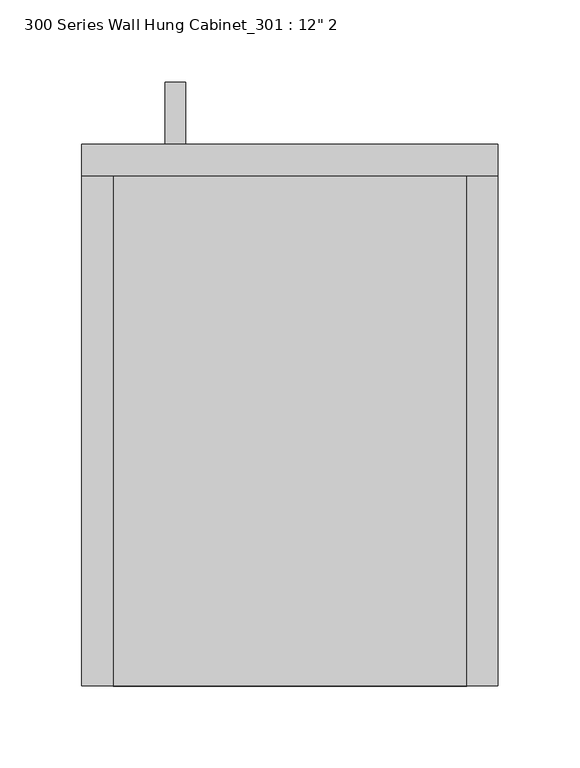
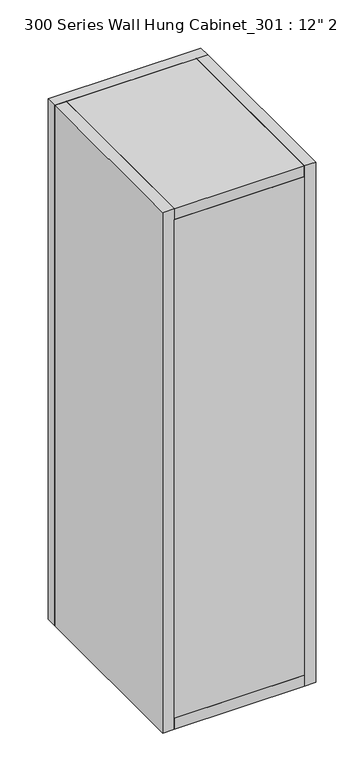
"""IFC4 building model written with IfcOpenShell, lengths in millimetres: furniture geometry."""

import ifcopenshell
import ifcopenshell.guid

model = None  # the IFC model being written
_history = None  # IfcOwnerHistory: only IFC2X3 demands one
_inside = {}  # id of a spatial element -> (the spatial element, [elements in it])
_under = {}  # id of a project, library or spatial element -> (it, [spatial elements below it])
_declared = {}  # id of a project -> (the project, [libraries it declares])
_typed = {}  # id of a type object -> (the type object, [elements of that type])
_made_of = {}  # id of a material, layer set ... -> (it, [elements and type objects made of it])


def new_model(schema):
    """Start an empty IFC model of exactly this schema.

    Asked for "IFC4X3", IfcOpenShell would pick the latest addendum, in which some entities
    have other attributes; the version numbers below select the first issue.
    IFC2X3 requires an IfcOwnerHistory on every rooted entity: one is made here for all.
    """
    global model, _history
    if schema == "IFC4X3":
        model = ifcopenshell.file(schema_version=(4, 3, 0, 0))
    else:
        model = ifcopenshell.file(schema=schema)
    _inside.clear()
    _under.clear()
    _declared.clear()
    _typed.clear()
    _made_of.clear()
    _history = None
    if model.schema == "IFC2X3":
        org = make("IfcOrganization", Name="unknown")
        user = make(
            "IfcPersonAndOrganization",
            ThePerson=make("IfcPerson", FamilyName="unknown"),
            TheOrganization=org,
        )
        app = make(
            "IfcApplication",
            ApplicationDeveloper=org,
            Version="unknown",
            ApplicationFullName="unknown",
            ApplicationIdentifier="unknown",
        )
        _history = make(
            "IfcOwnerHistory",
            OwningUser=user,
            OwningApplication=app,
            ChangeAction="ADDED",
            CreationDate=0,
        )
    return model


def make(cls, **values):
    """One entity of the class cls with the attributes given. An attribute that is None is left unset."""
    return model.create_entity(
        cls, **{name: value for name, value in values.items() if value is not None}
    )


def rooted(cls, **values):
    """An entity with a GlobalId (a new one), such as an element, a storey or a relation."""
    return make(cls, GlobalId=ifcopenshell.guid.new(), OwnerHistory=_history, **values)


def si_unit(unit_type, name, prefix=None):
    """IfcSIUnit, for example si_unit("LENGTHUNIT", "METRE", prefix="MILLI")."""
    return make("IfcSIUnit", UnitType=unit_type, Prefix=prefix, Name=name)


def assignment(units):
    """IfcUnitAssignment: the units of a project."""
    return None if units is None else make("IfcUnitAssignment", Units=units)


def point(xyz):
    """IfcCartesianPoint."""
    return None if xyz is None else make("IfcCartesianPoint", Coordinates=xyz)


def direction(xyz):
    """IfcDirection."""
    return None if xyz is None else make("IfcDirection", DirectionRatios=xyz)


def frame(location, z_axis=None, x_axis=None):
    """IfcAxis2Placement3D, a coordinate frame: its origin and axes. An axis left out is left unset."""
    return make(
        "IfcAxis2Placement3D",
        Location=point(location),
        Axis=direction(z_axis),
        RefDirection=direction(x_axis),
    )


def origin():
    """The frame at (0, 0, 0) with its axes left unset."""
    return frame((0.0, 0.0, 0.0))


def place(relative_to, where):
    """IfcLocalPlacement: puts the frame where relative to a parent placement (None: the world)."""
    return make(
        "IfcLocalPlacement", PlacementRelTo=relative_to, RelativePlacement=where
    )


def context(
    kind, dimensions, precision=None, world=None, true_north=None, identifier=None
):
    """IfcGeometricRepresentationContext, for example the 3D "Model" context."""
    return make(
        "IfcGeometricRepresentationContext",
        ContextIdentifier=identifier,
        ContextType=kind,
        CoordinateSpaceDimension=dimensions,
        Precision=precision,
        WorldCoordinateSystem=world,
        TrueNorth=true_north,
    )


def project(units=None, contexts=None):
    """IfcProject with its units and contexts."""
    return rooted(
        "IfcProject",
        Name="project",
        RepresentationContexts=contexts,
        UnitsInContext=assignment(units),
    )


def spatial(cls, under=None, at=None, **own):
    """A site, building, storey or space (cls), placed at a placement, below another one or the project."""
    s = rooted(cls, ObjectPlacement=at, **own)
    if under is not None:
        _under.setdefault(under.id(), (under, []))[1].append(s)
    return s


def polyline(points):
    """IfcPolyline through the points."""
    return make("IfcPolyline", Points=[point(p) for p in points])


def outline(outer, holes=None, kind="AREA"):
    """IfcArbitraryClosedProfileDef: a profile drawn as a closed curve; with holes, ...WithVoids."""
    if holes is None:
        return make("IfcArbitraryClosedProfileDef", ProfileType=kind, OuterCurve=outer)
    return make(
        "IfcArbitraryProfileDefWithVoids",
        ProfileType=kind,
        OuterCurve=outer,
        InnerCurves=holes,
    )


def extrude(swept, where, along, depth):
    """IfcExtrudedAreaSolid: the profile swept, set in the frame where, extruded along a direction by depth."""
    return make(
        "IfcExtrudedAreaSolid",
        SweptArea=swept,
        Position=where,
        ExtrudedDirection=direction(along),
        Depth=depth,
    )


def shape(context_of_items, identifier, shape_type, items):
    """IfcShapeRepresentation: the items that make up one representation, for example the "Body"."""
    return make(
        "IfcShapeRepresentation",
        ContextOfItems=context_of_items,
        RepresentationIdentifier=identifier,
        RepresentationType=shape_type,
        Items=items,
    )


def source(mapping_origin, context_of_items, identifier, shape_type, items):
    """IfcRepresentationMap: a shape defined once, which mapped items show again and again."""
    return make(
        "IfcRepresentationMap",
        MappingOrigin=mapping_origin,
        MappedRepresentation=shape(context_of_items, identifier, shape_type, items),
    )


def transform(
    local_origin,
    x_axis=None,
    y_axis=None,
    z_axis=None,
    scale=None,
    scale2=None,
    scale3=None,
    uniform=True,
):
    """IfcCartesianTransformationOperator3D, or its non-uniform kind. x_axis, y_axis, z_axis: its Axis1, 2, 3."""
    if uniform:
        return make(
            "IfcCartesianTransformationOperator3D",
            Axis1=direction(x_axis),
            Axis2=direction(y_axis),
            LocalOrigin=point(local_origin),
            Scale=scale,
            Axis3=direction(z_axis),
        )
    return make(
        "IfcCartesianTransformationOperator3DnonUniform",
        Axis1=direction(x_axis),
        Axis2=direction(y_axis),
        LocalOrigin=point(local_origin),
        Scale=scale,
        Axis3=direction(z_axis),
        Scale2=scale2,
        Scale3=scale3,
    )


def mapped(mapping_source, mapping_target):
    """IfcMappedItem: shows the shape of a source again, moved by a transform."""
    return make(
        "IfcMappedItem", MappingSource=mapping_source, MappingTarget=mapping_target
    )


def made_of(thing, what):
    """Note that an element or type object is made of a material, layer set ...; save() writes the relation."""
    if what is not None:
        _made_of.setdefault(what.id(), (what, []))[1].append(thing)
    return thing


def element(
    cls,
    number,
    at=None,
    inside=None,
    cuts=None,
    type_object=None,
    material=None,
    context=None,
    identifier="Body",
    shape_type=None,
    held_by="IfcProductDefinitionShape",
    body=None,
    shapes=None,
    **own,
):
    """One element of the class cls, such as IfcWall. Its Tag is "e" and its number.

    at: its placement. inside: the storey or other place that contains it. cuts: it is an
    opening in that element (IfcRelVoidsElement). A single representation is given by context,
    identifier, shape_type and body (its items); several are given by shapes. held_by: the class
    of the entity that holds the representations. save() writes the other relations.
    """
    e = rooted(cls, Tag="e%d" % number, ObjectPlacement=at, **own)
    if body is not None:
        shapes = [shape(context, identifier, shape_type, body)]
    if shapes is not None:
        e.Representation = make(held_by, Representations=shapes)
    if inside is not None:
        _inside.setdefault(inside.id(), (inside, []))[1].append(e)
    if cuts is not None:
        rooted(
            "IfcRelVoidsElement", RelatingBuildingElement=cuts, RelatedOpeningElement=e
        )
    if type_object is not None:
        _typed.setdefault(type_object.id(), (type_object, []))[1].append(e)
    return made_of(e, material)


def aggregate(whole, parts):
    """IfcRelAggregates: a whole, such as a stair, and the parts it consists of."""
    return rooted("IfcRelAggregates", RelatingObject=whole, RelatedObjects=parts)


def save(model, path):
    """Write the relations noted so far, then the file.

    IfcRelAggregates (storeys below a building ...), IfcRelContainedInSpatialStructure (elements
    in a storey), IfcRelDefinesByType, IfcRelAssociatesMaterial and IfcRelDeclares: one each for
    every whole, place, type object, material and project.
    """
    for whole, parts in _under.values():
        aggregate(whole, parts)
    for where, things in _inside.values():
        rooted(
            "IfcRelContainedInSpatialStructure",
            RelatedElements=things,
            RelatingStructure=where,
        )
    for kind, things in _typed.values():
        rooted("IfcRelDefinesByType", RelatedObjects=things, RelatingType=kind)
    for what, things in _made_of.values():
        rooted("IfcRelAssociatesMaterial", RelatedObjects=things, RelatingMaterial=what)
    for by, libraries in _declared.values():
        rooted("IfcRelDeclares", RelatingContext=by, RelatedDefinitions=libraries)
    model.write(path)


def furniture_bfdc1b7c(model_context):
    return source(origin(), model_context, "Body", "SweptSolid", [
        extrude(outline(polyline([(406.4, 1352.5425373), (406.4, 1365.2121874), (444.4810937, 1365.2121874), (444.4810937, 1270.0), (406.4, 1270.0), (406.4, 1282.6696501), (431.8114436, 1282.6696501), (431.8114436, 1352.5425373), (406.4, 1352.5425373)])), frame((-76.2, 0.0, 0.0), z_axis=(1.0, 0.0, 0.0), x_axis=(0.0, 1.0, 0.0)), (0.0, 0.0, 1.0), 12.4065288),
        extrude(outline(polyline([(107.95, 387.35), (107.95, 76.2), (-107.95, 76.2), (-107.95, 387.35), (107.95, 387.35)])), frame((0.0, 0.0, 1219.2), z_axis=(0.0, 0.0, 1.0), x_axis=(1.0, 0.0, 0.0)), (0.0, 0.0, 1.0), 19.05),
        extrude(outline(polyline([(107.95, 76.2), (-107.95, 76.2), (-107.95, 95.25), (107.95, 95.25), (107.95, 76.2)])), frame((0.0, 0.0, 1238.25), z_axis=(0.0, 0.0, 1.0), x_axis=(1.0, 0.0, 0.0)), (0.0, 0.0, 1.0), 876.3),
        extrude(outline(polyline([(127.0, 387.35), (-127.0, 387.35), (-127.0, 406.4), (127.0, 406.4), (127.0, 387.35)])), frame((0.0, 0.0, 1219.2), z_axis=(0.0, 0.0, 1.0), x_axis=(1.0, 0.0, 0.0)), (0.0, 0.0, 1.0), 914.4),
        extrude(outline(polyline([(-127.0, 76.2), (-127.0, 387.35), (-107.95, 387.35), (-107.95, 76.2), (-127.0, 76.2)])), frame((0.0, 0.0, 1219.2), z_axis=(0.0, 0.0, 1.0), x_axis=(1.0, 0.0, 0.0)), (0.0, 0.0, 1.0), 914.4),
        extrude(outline(polyline([(107.95, 76.2), (107.95, 387.35), (127.0, 387.35), (127.0, 76.2), (107.95, 76.2)])), frame((0.0, 0.0, 1219.2), z_axis=(0.0, 0.0, 1.0), x_axis=(1.0, 0.0, 0.0)), (0.0, 0.0, 1.0), 914.4),
        extrude(outline(polyline([(107.95, 387.35), (107.95, 76.2), (-107.95, 76.2), (-107.95, 387.35), (107.95, 387.35)])), frame((0.0, 0.0, 2114.55), z_axis=(0.0, 0.0, 1.0), x_axis=(1.0, 0.0, 0.0)), (0.0, 0.0, 1.0), 19.05),
    ])


if __name__ == "__main__":
    model = new_model("IFC4")
    model_context = context("Model", 3, world=origin())
    ifc_project = project(units=[si_unit("LENGTHUNIT", "METRE", prefix="MILLI")], contexts=[model_context])
    site = spatial("IfcSite", under=ifc_project)
    building = spatial("IfcBuilding", under=site)
    placement = place(None, origin())
    furniture_shape = furniture_bfdc1b7c(model_context)
    element("IfcFurniture", 1, ObjectType="300 Series Wall Hung Cabinet_301 : 12\" 2", at=placement, inside=building, context=model_context, shape_type="MappedRepresentation", body=[
        mapped(furniture_shape, transform((0.0, 0.0, 0.0), x_axis=(1.0, 0.0, 0.0), y_axis=(0.0, 1.0, 0.0), z_axis=(0.0, 0.0, 1.0))),
    ])
    save(model, "model.ifc")

# Revit data of these elements
# Type "300 Series Wall Hung Cabinet_301 : 12\" 2"
#   URL = "www.wicnet.org/manual_sections.asp"
#   Model = "301"
#   Manufacturer = "Woodwork Institute"
#   Description = "Wall Hung Cabinet"
#   Content Creator URL = "www.AECcontent.com"
#   Content Creator = "AECcontent"
#   Assembly Code = "E2010200"
#   Width = 0' - 10"
#   Top of Cabinet = 7' - 0"
#   Height = 3' - 0"
#   Depth = 1' - 1"
#   Top Panel Material = Cabinet
#   Side Panel Material = Cabinet
#   Door Panel Material = Cabinet
#   Shelf Panel Material = Cabinet
# Element 1 (IfcFurniture, "300 Series Wall Hung Cabinet_301 : 12\" 2")
#   Materials on its faces: "Cabinet", "Default metal"
# Materials
#   "Cabinet": class "Wood", colour RGB 189 170 130, transparency 0, Cost = 0
#   "Default metal": class "Unassigned", colour RGB 204 204 204, transparency 0
